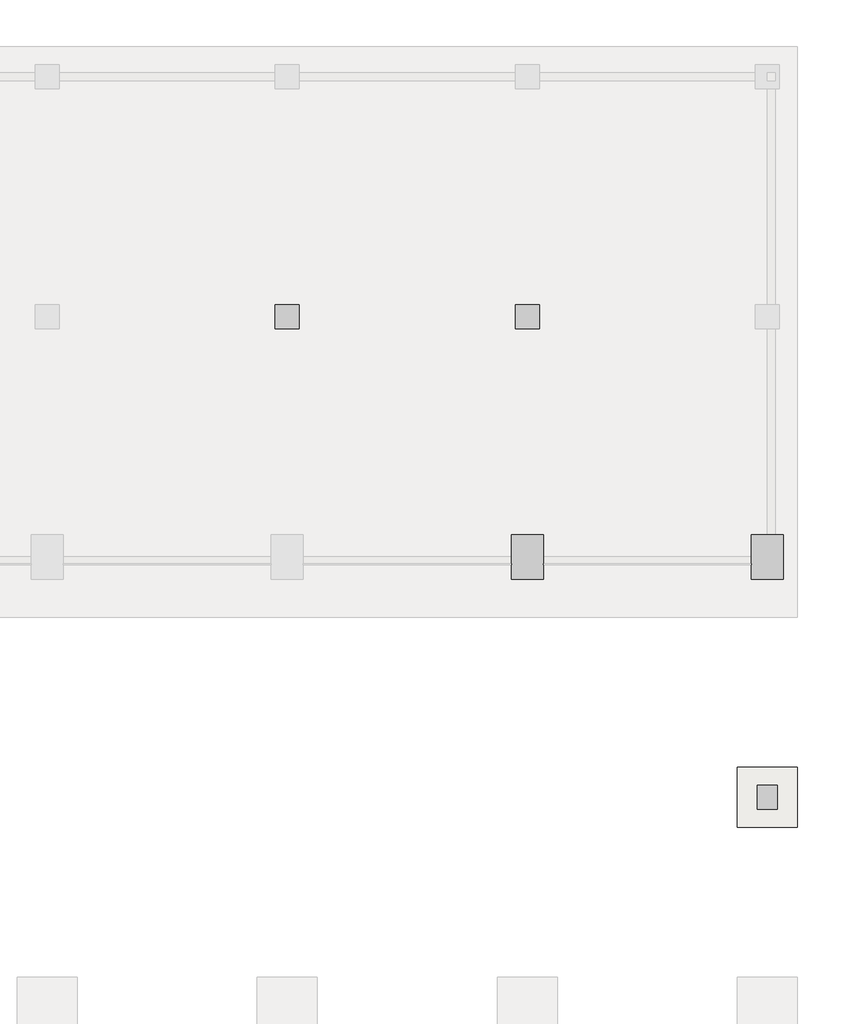
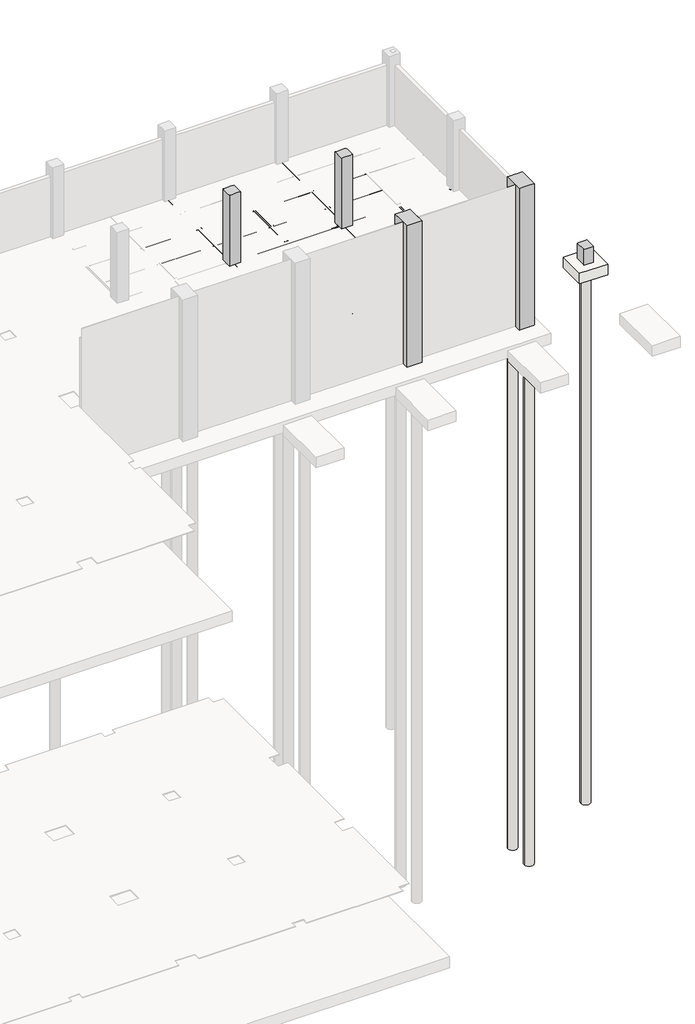
# Not in any storey, part 15 of 16: 29 beams, 5 columns, 4 slabs.
# Revit data of these elements (continued)
# Elements 30, 31 (IfcColumn, "RC_Column_Rectangular : H_SC_AR_S15_UG PED_Bit_800x1100_PD1") (continued)
#   Structural Material = 00_Concrete_Reinf. Conc.
#   Phase Created = New Construction
#   Materials on its faces: "00_Concrete_Reinf. Conc."
# Element 32 (IfcColumn, "RC_Column_Rectangular : H_SC_AR_S15_UG PED_Bit_500x600_PD2")
#   Comments = ""
#   hec_material3 = none
#   hec_material2 = none
#   hec_material1 = none
#   Structural Material = 00_Concrete_Reinf. Conc.
#   Phase Created = New Construction
#   Materials on its faces: "00_Concrete_Reinf. Conc."
# Elements 33, 34 (IfcColumn, "RC_Column_Rectangular : H_SC_AR_S15_UG PED_Bit_600x600_BC1")
#   Comments = ""
#   hec_material3 = none
#   hec_material2 = none
#   hec_material1 = none
#   Structural Material = 00_Concrete_Reinf. Conc.
#   Phase Created = New Construction
#   Materials on its faces: "00_Concrete_Reinf. Conc."
# Element 35 (IfcSlab, "Foundation Rectangular (Non-Pile) : H_SF_AR_S18_Shallow Fdn_Bitumen_1500x1500xT600_F2")
#   Structural Material = 00_Concrete_Reinf. Conc.
#   Phase Created = New Construction
#   Materials on its faces: "00_Concrete_Reinf. Conc."
# Element 36 (IfcSlab, "PILE : H_SF_AR_S19_PHC Pile_Pre-boring_D500_L30")
#   Structural Material = Concrete, Precast
#   Phase Created = New Construction
#   Materials on its faces: "Concrete, Precast"
# Elements 37, 38 (IfcSlab, "PILE : H_SF_AR_S19_PHC Pile_Pre-boring_D500_L30")
#   Structural Material = none
#   Phase Created = New Construction
# Materials
#   "Steel, 45-345": class "Metal", colour RGB 189 187 185, transparency 0, Description = "Steel 345 MPa", Cost = 0
#   "00_Concrete_Reinf. Conc.": class "Concrete", colour RGB 176 176 176, transparency 0, Description = "Reinf. Conc.", Cost = 0, Image = Concrete.Cast-In-Place.Flat.Polished.Grey.jpg
#   "Concrete, Precast": class "Concrete", colour RGB 115 116 108, transparency 0, Description = "Precast concrete", Cost = 0
